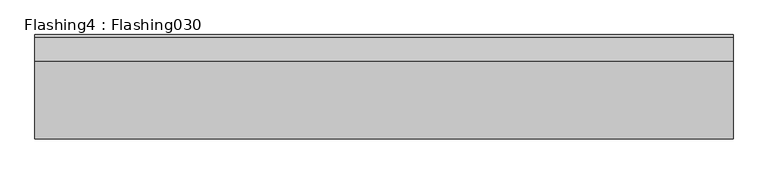
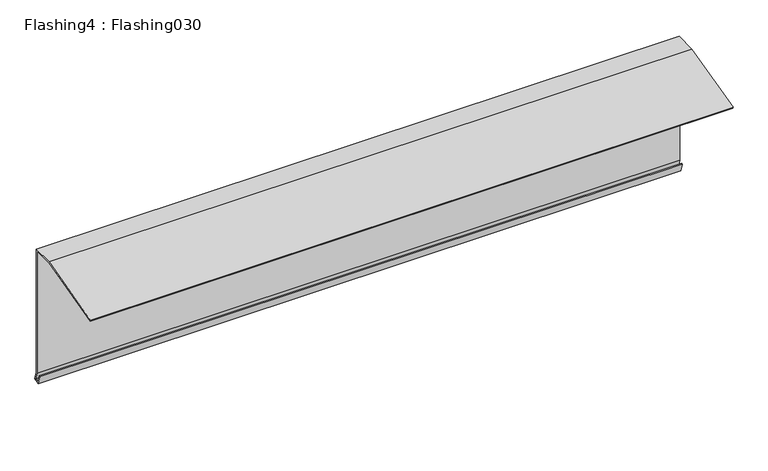
"""IFC4 building model written with IfcOpenShell, lengths in millimetres: proxy geometry, Flashing4 : Flashing030."""

from ifc_helpers import new_model, si_unit, frame, origin, place, context, project, spatial, polyline, outline, extrude, source, transform, mapped, element, save


def flashing4_flashing030_b08d50d1(model_context):
    return source(origin(), model_context, "Body", "SweptSolid", [
        extrude(outline(polyline([(10761.7798572, 43905.1238578), (10830.6026166, 43905.1238578), (10830.6026166, 43500.7036908), (10838.8883656, 43473.7122248), (10821.3263764, 43468.3211047), (10812.8048921, 43495.8445422), (10816.6259444, 43497.0275717), (10823.9688462, 43473.3108235), (10833.8963841, 43476.3435481), (10826.6026166, 43500.1035576), (10826.6026166, 43901.1238578), (10762.2827517, 43901.1238578), (10540.7821389, 43844.5336305), (10539.7920001, 43848.4091467), (10761.7798572, 43905.1238578)])), frame((3627.1902954, 0.0, 0.0), z_axis=(1.0, 0.0, 0.0), x_axis=(0.0, 1.0, 0.0)), (0.0, 0.0, 1.0), 1999.85),
    ])


if __name__ == "__main__":
    model = new_model("IFC4")
    model_context = context("Model", 3, world=origin())
    ifc_project = project(units=[si_unit("LENGTHUNIT", "METRE", prefix="MILLI")], contexts=[model_context])
    site = spatial("IfcSite", under=ifc_project)
    building = spatial("IfcBuilding", under=site)
    placement = place(None, origin())
    flashing4_flashing030_shape = flashing4_flashing030_b08d50d1(model_context)
    element("IfcBuildingElementProxy", 1, Name="Flashing4 : Flashing030", ObjectType="Flashing4 : Flashing030", at=placement, inside=building, context=model_context, shape_type="MappedRepresentation", body=[
        mapped(flashing4_flashing030_shape, transform((0.0, 0.0, 0.0), x_axis=(1.0, 0.0, 0.0), y_axis=(0.0, 1.0, 0.0), z_axis=(0.0, 0.0, 1.0))),
    ])
    save(model, "model.ifc")

# Revit data of these elements
# Type "Flashing4 : Flashing030"
#   NameOverride = "Flashing030"
# Element 1 (IfcBuildingElementProxy, "Flashing4 : Flashing030")
#   Materials on its faces: "BRAKE METAL EAVE TRIM TO MATCH STANDING SEAM COLOR"
# Materials
#   "BRAKE METAL EAVE TRIM TO MATCH STANDING SEAM COLOR": class "Unassigned", colour RGB 128 128 128, transparency 0, Cost = 0
